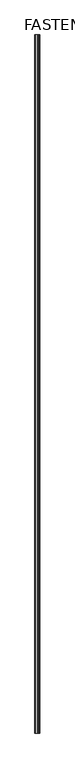
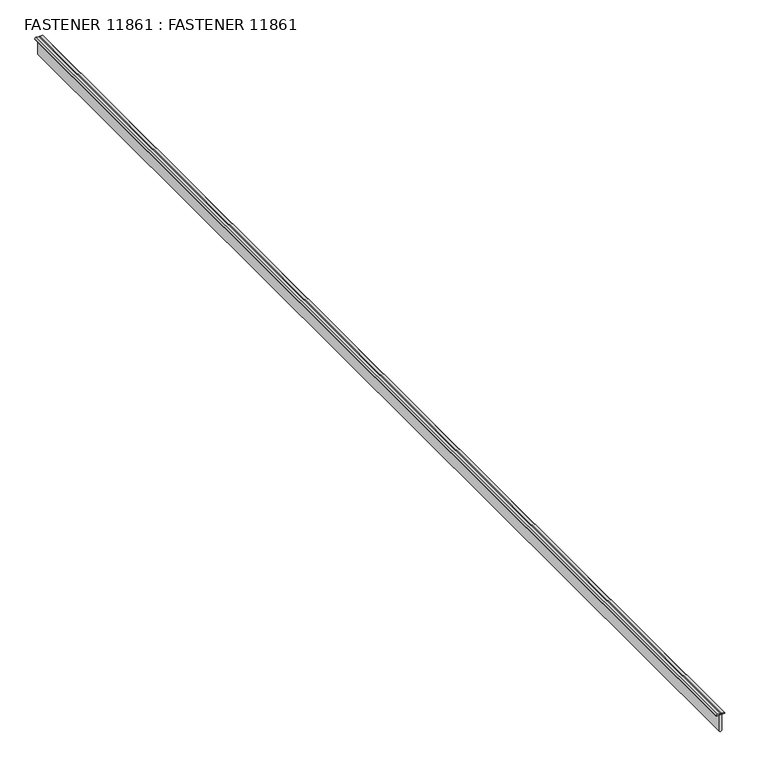
"""IFC4 building model written with IfcOpenShell, lengths in millimetres: proxy geometry, FASTENER 11861 : FASTENER 11861."""

import ifcopenshell
import ifcopenshell.guid

model = None  # the IFC model being written
_history = None  # IfcOwnerHistory: only IFC2X3 demands one
_inside = {}  # id of a spatial element -> (the spatial element, [elements in it])
_under = {}  # id of a project, library or spatial element -> (it, [spatial elements below it])
_declared = {}  # id of a project -> (the project, [libraries it declares])
_typed = {}  # id of a type object -> (the type object, [elements of that type])
_made_of = {}  # id of a material, layer set ... -> (it, [elements and type objects made of it])


def new_model(schema):
    """Start an empty IFC model of exactly this schema.

    Asked for "IFC4X3", IfcOpenShell would pick the latest addendum, in which some entities
    have other attributes; the version numbers below select the first issue.
    IFC2X3 requires an IfcOwnerHistory on every rooted entity: one is made here for all.
    """
    global model, _history
    if schema == "IFC4X3":
        model = ifcopenshell.file(schema_version=(4, 3, 0, 0))
    else:
        model = ifcopenshell.file(schema=schema)
    _inside.clear()
    _under.clear()
    _declared.clear()
    _typed.clear()
    _made_of.clear()
    _history = None
    if model.schema == "IFC2X3":
        org = make("IfcOrganization", Name="unknown")
        user = make(
            "IfcPersonAndOrganization",
            ThePerson=make("IfcPerson", FamilyName="unknown"),
            TheOrganization=org,
        )
        app = make(
            "IfcApplication",
            ApplicationDeveloper=org,
            Version="unknown",
            ApplicationFullName="unknown",
            ApplicationIdentifier="unknown",
        )
        _history = make(
            "IfcOwnerHistory",
            OwningUser=user,
            OwningApplication=app,
            ChangeAction="ADDED",
            CreationDate=0,
        )
    return model


def make(cls, **values):
    """One entity of the class cls with the attributes given. An attribute that is None is left unset."""
    return model.create_entity(
        cls, **{name: value for name, value in values.items() if value is not None}
    )


def rooted(cls, **values):
    """An entity with a GlobalId (a new one), such as an element, a storey or a relation."""
    return make(cls, GlobalId=ifcopenshell.guid.new(), OwnerHistory=_history, **values)


def si_unit(unit_type, name, prefix=None):
    """IfcSIUnit, for example si_unit("LENGTHUNIT", "METRE", prefix="MILLI")."""
    return make("IfcSIUnit", UnitType=unit_type, Prefix=prefix, Name=name)


def assignment(units):
    """IfcUnitAssignment: the units of a project."""
    return None if units is None else make("IfcUnitAssignment", Units=units)


def point(xyz):
    """IfcCartesianPoint."""
    return None if xyz is None else make("IfcCartesianPoint", Coordinates=xyz)


def direction(xyz):
    """IfcDirection."""
    return None if xyz is None else make("IfcDirection", DirectionRatios=xyz)


def frame(location, z_axis=None, x_axis=None):
    """IfcAxis2Placement3D, a coordinate frame: its origin and axes. An axis left out is left unset."""
    return make(
        "IfcAxis2Placement3D",
        Location=point(location),
        Axis=direction(z_axis),
        RefDirection=direction(x_axis),
    )


def origin():
    """The frame at (0, 0, 0) with its axes left unset."""
    return frame((0.0, 0.0, 0.0))


def place(relative_to, where):
    """IfcLocalPlacement: puts the frame where relative to a parent placement (None: the world)."""
    return make(
        "IfcLocalPlacement", PlacementRelTo=relative_to, RelativePlacement=where
    )


def context(
    kind, dimensions, precision=None, world=None, true_north=None, identifier=None
):
    """IfcGeometricRepresentationContext, for example the 3D "Model" context."""
    return make(
        "IfcGeometricRepresentationContext",
        ContextIdentifier=identifier,
        ContextType=kind,
        CoordinateSpaceDimension=dimensions,
        Precision=precision,
        WorldCoordinateSystem=world,
        TrueNorth=true_north,
    )


def project(units=None, contexts=None):
    """IfcProject with its units and contexts."""
    return rooted(
        "IfcProject",
        Name="project",
        RepresentationContexts=contexts,
        UnitsInContext=assignment(units),
    )


def spatial(cls, under=None, at=None, **own):
    """A site, building, storey or space (cls), placed at a placement, below another one or the project."""
    s = rooted(cls, ObjectPlacement=at, **own)
    if under is not None:
        _under.setdefault(under.id(), (under, []))[1].append(s)
    return s


def polyline(points):
    """IfcPolyline through the points."""
    return make("IfcPolyline", Points=[point(p) for p in points])


def outline(outer, holes=None, kind="AREA"):
    """IfcArbitraryClosedProfileDef: a profile drawn as a closed curve; with holes, ...WithVoids."""
    if holes is None:
        return make("IfcArbitraryClosedProfileDef", ProfileType=kind, OuterCurve=outer)
    return make(
        "IfcArbitraryProfileDefWithVoids",
        ProfileType=kind,
        OuterCurve=outer,
        InnerCurves=holes,
    )


def extrude(swept, where, along, depth):
    """IfcExtrudedAreaSolid: the profile swept, set in the frame where, extruded along a direction by depth."""
    return make(
        "IfcExtrudedAreaSolid",
        SweptArea=swept,
        Position=where,
        ExtrudedDirection=direction(along),
        Depth=depth,
    )


def shape(context_of_items, identifier, shape_type, items):
    """IfcShapeRepresentation: the items that make up one representation, for example the "Body"."""
    return make(
        "IfcShapeRepresentation",
        ContextOfItems=context_of_items,
        RepresentationIdentifier=identifier,
        RepresentationType=shape_type,
        Items=items,
    )


def source(mapping_origin, context_of_items, identifier, shape_type, items):
    """IfcRepresentationMap: a shape defined once, which mapped items show again and again."""
    return make(
        "IfcRepresentationMap",
        MappingOrigin=mapping_origin,
        MappedRepresentation=shape(context_of_items, identifier, shape_type, items),
    )


def transform(
    local_origin,
    x_axis=None,
    y_axis=None,
    z_axis=None,
    scale=None,
    scale2=None,
    scale3=None,
    uniform=True,
):
    """IfcCartesianTransformationOperator3D, or its non-uniform kind. x_axis, y_axis, z_axis: its Axis1, 2, 3."""
    if uniform:
        return make(
            "IfcCartesianTransformationOperator3D",
            Axis1=direction(x_axis),
            Axis2=direction(y_axis),
            LocalOrigin=point(local_origin),
            Scale=scale,
            Axis3=direction(z_axis),
        )
    return make(
        "IfcCartesianTransformationOperator3DnonUniform",
        Axis1=direction(x_axis),
        Axis2=direction(y_axis),
        LocalOrigin=point(local_origin),
        Scale=scale,
        Axis3=direction(z_axis),
        Scale2=scale2,
        Scale3=scale3,
    )


def mapped(mapping_source, mapping_target):
    """IfcMappedItem: shows the shape of a source again, moved by a transform."""
    return make(
        "IfcMappedItem", MappingSource=mapping_source, MappingTarget=mapping_target
    )


def made_of(thing, what):
    """Note that an element or type object is made of a material, layer set ...; save() writes the relation."""
    if what is not None:
        _made_of.setdefault(what.id(), (what, []))[1].append(thing)
    return thing


def element(
    cls,
    number,
    at=None,
    inside=None,
    cuts=None,
    type_object=None,
    material=None,
    context=None,
    identifier="Body",
    shape_type=None,
    held_by="IfcProductDefinitionShape",
    body=None,
    shapes=None,
    **own,
):
    """One element of the class cls, such as IfcWall. Its Tag is "e" and its number.

    at: its placement. inside: the storey or other place that contains it. cuts: it is an
    opening in that element (IfcRelVoidsElement). A single representation is given by context,
    identifier, shape_type and body (its items); several are given by shapes. held_by: the class
    of the entity that holds the representations. save() writes the other relations.
    """
    e = rooted(cls, Tag="e%d" % number, ObjectPlacement=at, **own)
    if body is not None:
        shapes = [shape(context, identifier, shape_type, body)]
    if shapes is not None:
        e.Representation = make(held_by, Representations=shapes)
    if inside is not None:
        _inside.setdefault(inside.id(), (inside, []))[1].append(e)
    if cuts is not None:
        rooted(
            "IfcRelVoidsElement", RelatingBuildingElement=cuts, RelatedOpeningElement=e
        )
    if type_object is not None:
        _typed.setdefault(type_object.id(), (type_object, []))[1].append(e)
    return made_of(e, material)


def aggregate(whole, parts):
    """IfcRelAggregates: a whole, such as a stair, and the parts it consists of."""
    return rooted("IfcRelAggregates", RelatingObject=whole, RelatedObjects=parts)


def save(model, path):
    """Write the relations noted so far, then the file.

    IfcRelAggregates (storeys below a building ...), IfcRelContainedInSpatialStructure (elements
    in a storey), IfcRelDefinesByType, IfcRelAssociatesMaterial and IfcRelDeclares: one each for
    every whole, place, type object, material and project.
    """
    for whole, parts in _under.values():
        aggregate(whole, parts)
    for where, things in _inside.values():
        rooted(
            "IfcRelContainedInSpatialStructure",
            RelatedElements=things,
            RelatingStructure=where,
        )
    for kind, things in _typed.values():
        rooted("IfcRelDefinesByType", RelatedObjects=things, RelatingType=kind)
    for what, things in _made_of.values():
        rooted("IfcRelAssociatesMaterial", RelatedObjects=things, RelatingMaterial=what)
    for by, libraries in _declared.values():
        rooted("IfcRelDeclares", RelatingContext=by, RelatedDefinitions=libraries)
    model.write(path)


def fastener_11861_fastener_11861_40db04d7(model_context):
    return source(origin(), model_context, "Body", "SweptSolid", [
        extrude(outline(polyline([(42551.3049701, 5981.517626), (42579.6987049, 5981.517626), (42579.6987049, 5977.3107075), (42550.7399648, 5977.3107075), (42549.1244121, 5978.9677221), (42551.3049701, 5981.517626)])), frame((0.0, -1052.8906574, 0.0), z_axis=(0.0, 1.0, 0.0), x_axis=(0.0, 0.0, 1.0)), (0.0, 0.0, 1.0), 1999.85),
        extrude(outline(polyline([(42580.5349921, 5972.2779845), (42579.6987049, 5972.2671879), (42579.6987049, 5986.5634932), (42580.508527, 5986.5634932), (42582.1023984, 5985.3247911), (42582.1023984, 5980.4457092), (42580.1167322, 5980.0391089), (42580.1167322, 5978.792004), (42581.7222633, 5978.792004), (42582.1288635, 5973.5166866), (42580.5349921, 5972.2779845)])), frame((0.0, -1052.8906574, 0.0), z_axis=(0.0, 1.0, 0.0), x_axis=(0.0, 0.0, 1.0)), (0.0, 0.0, 1.0), 1999.85),
    ])


if __name__ == "__main__":
    model = new_model("IFC4")
    model_context = context("Model", 3, world=origin())
    ifc_project = project(units=[si_unit("LENGTHUNIT", "METRE", prefix="MILLI")], contexts=[model_context])
    site = spatial("IfcSite", under=ifc_project)
    building = spatial("IfcBuilding", under=site)
    placement = place(None, origin())
    fastener_11861_fastener_11861_shape = fastener_11861_fastener_11861_40db04d7(model_context)
    element("IfcBuildingElementProxy", 1, Name="FASTENER 11861 : FASTENER 11861", ObjectType="FASTENER 11861 : FASTENER 11861", at=placement, inside=building, context=model_context, shape_type="MappedRepresentation", body=[
        mapped(fastener_11861_fastener_11861_shape, transform((0.0, 0.0, 0.0), x_axis=(1.0, 0.0, 0.0), y_axis=(0.0, 1.0, 0.0), z_axis=(0.0, 0.0, 1.0))),
    ])
    save(model, "model.ifc")

# Revit data of these elements
# Type "FASTENER 11861 : FASTENER 11861"
#   NameOverride = "FASTENER"
# Element 1 (IfcBuildingElementProxy, "FASTENER 11861 : FASTENER 11861")
#   Materials on its faces: "ENGINEERED PANCAKE HEAD FASTENER @ 12\" O.C."
# Materials
#   "ENGINEERED PANCAKE HEAD FASTENER @ 12\" O.C.": class "Unassigned", colour RGB 255 255 255, transparency 0, Cost = 0
